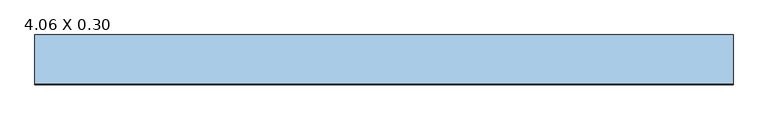
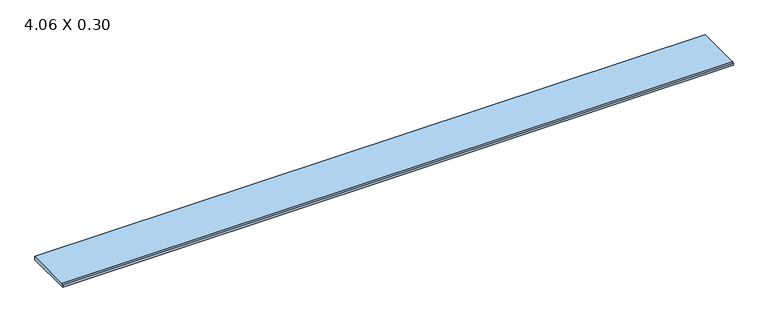
"""IFC4 building model written with IfcOpenShell, lengths in millimetres: window geometry, .CC_ND 300_PEDRA_PEITORIL RETO : 4.06 X 0.30."""

from ifc_helpers import new_model, si_unit, point, frame, frame_2d, origin, place, context, project, spatial, polyline, circle_curve, trimmed, segment, composite_curve, outline, extrude, source, transform, mapped, element, save


def window_4_06_x_0_30_b1d56b02(model_context):
    return source(origin(), model_context, "Body", "SweptSolid", [
        extrude(outline(composite_curve([segment(polyline([(-144.4083081, 1480.0), (-144.4083081, 1488.1993124), (-149.1619526, 1488.1993124), (-149.1619526, 1480.0), (-159.9, 1480.0), (-159.9, 1493.3808343)]), True, "CONTINUOUS"), segment(trimmed(circle_curve(frame_2d((-153.2808343, 1493.3808343)), 6.6191657), [point((-159.9, 1493.3808343))], [point((-153.2808343, 1500.0))], False, "CARTESIAN"), True, "CONTINUOUS"), segment(polyline([(-153.2808343, 1500.0), (129.9, 1500.0), (129.9, 1480.0), (-144.4083081, 1480.0)]), True, "CONTINUOUS")], self_intersect=False)), frame((-2030.0, 0.0, 0.0), z_axis=(1.0, 0.0, 0.0), x_axis=(0.0, 1.0, 0.0)), (0.0, 0.0, 1.0), 4060.0),
    ])


if __name__ == "__main__":
    model = new_model("IFC4")
    model_context = context("Model", 3, world=origin())
    ifc_project = project(units=[si_unit("LENGTHUNIT", "METRE", prefix="MILLI")], contexts=[model_context])
    site = spatial("IfcSite", under=ifc_project)
    building = spatial("IfcBuilding", under=site)
    placement = place(None, origin())
    window_4_06_x_0_30_shape = window_4_06_x_0_30_b1d56b02(model_context)
    element("IfcWindow", 1, ObjectType=".CC_ND 300_PEDRA_PEITORIL RETO : 4.06 X 0.30", at=placement, inside=building, context=model_context, shape_type="MappedRepresentation", body=[
        mapped(window_4_06_x_0_30_shape, transform((0.0, 0.0, 0.0), x_axis=(1.0, 0.0, 0.0), y_axis=(0.0, 1.0, 0.0), z_axis=(0.0, 0.0, 1.0))),
    ])
    save(model, "model.ifc")

# Revit data of these elements
# Type ".CC_ND 300_PEDRA_PEITORIL RETO : 4.06 X 0.30"
#   Type Mark = "72"
#   Largura da pedra [instance default] = 0.26 m
#   Extensão interior peitoril [instance default] = 0.03 m
#   Extensão exterior peitoril [instance default] = 0.03 m
#   Espessura = 0.02 m
#   Comprimento = 4.06 m
#   Altura-padrão do peitoril = 1.48 m
#   Peitoril = .GRANITO_BRANCO_ITAUNAS
#   Rough Width = 0
#   Rough Height = 0
#   Height = 0
#   Wall Closure = (empty or 0)
#   Width = 0
# Element 1 (IfcWindow, ".CC_ND 300_PEDRA_PEITORIL RETO : 4.06 X 0.30")
#   Largura da pedra = 0.2898 m
#   Extensão interior peitoril = 0.00 m
#   Materials on its faces: ".GRANITO_BRANCO_ITAUNAS"
# Materials
#   ".GRANITO_BRANCO_ITAUNAS": class ".CC_PEDRA REVEST.", colour RGB 202 195 174, transparency 0, Description = "Revestimento em granito", Cost = 0
